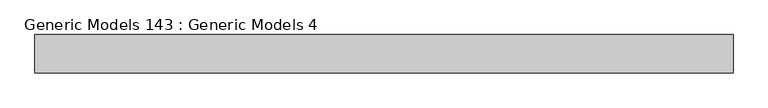
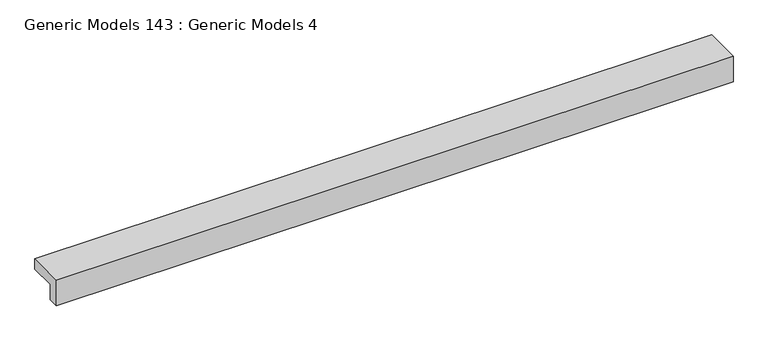
"""IFC4 building model written with IfcOpenShell, lengths in millimetres: proxy geometry, Generic Models 143 : Generic Models 4."""

from ifc_helpers import new_model, si_unit, frame, origin, place, context, project, spatial, polyline, outline, extrude, source, transform, mapped, element, save


def generic_models_143_generic_models_4_e6e117fe(model_context):
    return source(origin(), model_context, "Body", "SweptSolid", [
        extrude(outline(polyline([(6851.0769662, 124173.996), (7543.2269662, 124173.996), (7543.2269662, 123970.796), (7054.2769662, 123970.796), (7054.2769662, 123675.2519226), (6851.0769662, 123675.2519226), (6851.0769662, 124173.996)])), frame((-287.5914237, 0.0, 0.0), z_axis=(1.0, 0.0, 0.0), x_axis=(0.0, 1.0, 0.0)), (0.0, 0.0, 1.0), 12547.6),
    ])


if __name__ == "__main__":
    model = new_model("IFC4")
    model_context = context("Model", 3, world=origin())
    ifc_project = project(units=[si_unit("LENGTHUNIT", "METRE", prefix="MILLI")], contexts=[model_context])
    site = spatial("IfcSite", under=ifc_project)
    building = spatial("IfcBuilding", under=site)
    placement = place(None, origin())
    generic_models_143_generic_models_4_shape = generic_models_143_generic_models_4_e6e117fe(model_context)
    element("IfcBuildingElementProxy", 1, Name="Generic Models 143 : Generic Models 4", ObjectType="Generic Models 143 : Generic Models 4", at=placement, inside=building, context=model_context, shape_type="MappedRepresentation", body=[
        mapped(generic_models_143_generic_models_4_shape, transform((0.0, 0.0, 0.0), x_axis=(1.0, 0.0, 0.0), y_axis=(0.0, 1.0, 0.0), z_axis=(0.0, 0.0, 1.0))),
    ])
    save(model, "model.ifc")

# Revit data of these elements
# Element 1 (IfcBuildingElementProxy, "Generic Models 143 : Generic Models 4")
#   Materials on its faces: "_ 8\" CONCRETE SLAB W/ GRADE BEAM (SEE STRUCT. DWGS)(1)"
# Materials
#   "_ 8\" CONCRETE SLAB W/ GRADE BEAM (SEE STRUCT. DWGS)(1)": class "Generic", colour RGB 191 191 191, transparency 0, Cost = 0
